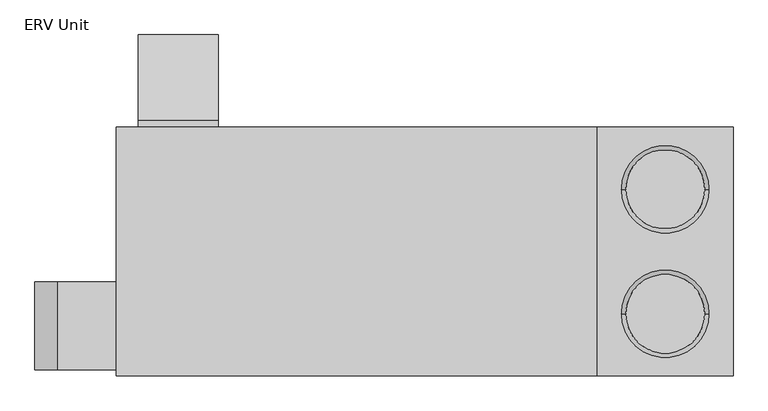
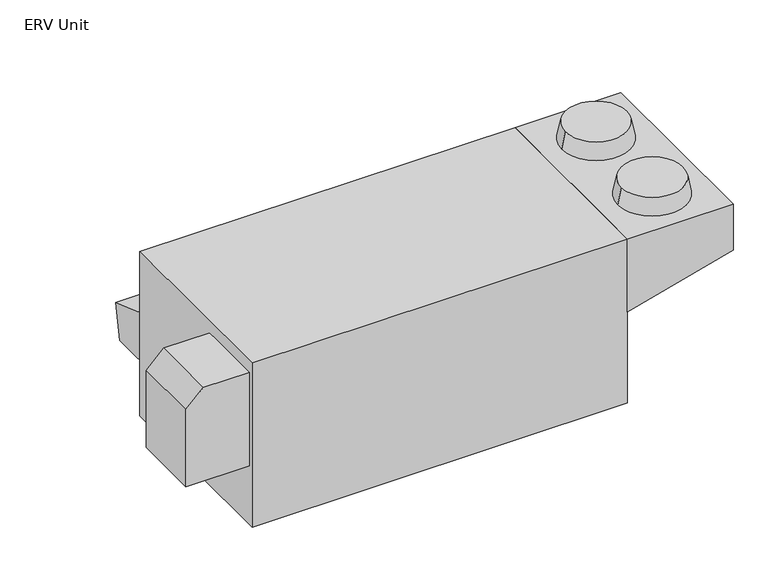
"""IFC4 building model written with IfcOpenShell, lengths in millimetres: proxy geometry, Energy Recovery-ER_H : ERV Unit."""

import ifcopenshell
import ifcopenshell.guid

model = None  # the IFC model being written
_history = None  # IfcOwnerHistory: only IFC2X3 demands one
_inside = {}  # id of a spatial element -> (the spatial element, [elements in it])
_under = {}  # id of a project, library or spatial element -> (it, [spatial elements below it])
_declared = {}  # id of a project -> (the project, [libraries it declares])
_typed = {}  # id of a type object -> (the type object, [elements of that type])
_made_of = {}  # id of a material, layer set ... -> (it, [elements and type objects made of it])


def new_model(schema):
    """Start an empty IFC model of exactly this schema.

    Asked for "IFC4X3", IfcOpenShell would pick the latest addendum, in which some entities
    have other attributes; the version numbers below select the first issue.
    IFC2X3 requires an IfcOwnerHistory on every rooted entity: one is made here for all.
    """
    global model, _history
    if schema == "IFC4X3":
        model = ifcopenshell.file(schema_version=(4, 3, 0, 0))
    else:
        model = ifcopenshell.file(schema=schema)
    _inside.clear()
    _under.clear()
    _declared.clear()
    _typed.clear()
    _made_of.clear()
    _history = None
    if model.schema == "IFC2X3":
        org = make("IfcOrganization", Name="unknown")
        user = make(
            "IfcPersonAndOrganization",
            ThePerson=make("IfcPerson", FamilyName="unknown"),
            TheOrganization=org,
        )
        app = make(
            "IfcApplication",
            ApplicationDeveloper=org,
            Version="unknown",
            ApplicationFullName="unknown",
            ApplicationIdentifier="unknown",
        )
        _history = make(
            "IfcOwnerHistory",
            OwningUser=user,
            OwningApplication=app,
            ChangeAction="ADDED",
            CreationDate=0,
        )
    return model


def make(cls, **values):
    """One entity of the class cls with the attributes given. An attribute that is None is left unset."""
    return model.create_entity(
        cls, **{name: value for name, value in values.items() if value is not None}
    )


def rooted(cls, **values):
    """An entity with a GlobalId (a new one), such as an element, a storey or a relation."""
    return make(cls, GlobalId=ifcopenshell.guid.new(), OwnerHistory=_history, **values)


def si_unit(unit_type, name, prefix=None):
    """IfcSIUnit, for example si_unit("LENGTHUNIT", "METRE", prefix="MILLI")."""
    return make("IfcSIUnit", UnitType=unit_type, Prefix=prefix, Name=name)


def assignment(units):
    """IfcUnitAssignment: the units of a project."""
    return None if units is None else make("IfcUnitAssignment", Units=units)


def point(xyz):
    """IfcCartesianPoint."""
    return None if xyz is None else make("IfcCartesianPoint", Coordinates=xyz)


def direction(xyz):
    """IfcDirection."""
    return None if xyz is None else make("IfcDirection", DirectionRatios=xyz)


def frame(location, z_axis=None, x_axis=None):
    """IfcAxis2Placement3D, a coordinate frame: its origin and axes. An axis left out is left unset."""
    return make(
        "IfcAxis2Placement3D",
        Location=point(location),
        Axis=direction(z_axis),
        RefDirection=direction(x_axis),
    )


def origin():
    """The frame at (0, 0, 0) with its axes left unset."""
    return frame((0.0, 0.0, 0.0))


def place(relative_to, where):
    """IfcLocalPlacement: puts the frame where relative to a parent placement (None: the world)."""
    return make(
        "IfcLocalPlacement", PlacementRelTo=relative_to, RelativePlacement=where
    )


def context(
    kind, dimensions, precision=None, world=None, true_north=None, identifier=None
):
    """IfcGeometricRepresentationContext, for example the 3D "Model" context."""
    return make(
        "IfcGeometricRepresentationContext",
        ContextIdentifier=identifier,
        ContextType=kind,
        CoordinateSpaceDimension=dimensions,
        Precision=precision,
        WorldCoordinateSystem=world,
        TrueNorth=true_north,
    )


def project(units=None, contexts=None):
    """IfcProject with its units and contexts."""
    return rooted(
        "IfcProject",
        Name="project",
        RepresentationContexts=contexts,
        UnitsInContext=assignment(units),
    )


def spatial(cls, under=None, at=None, **own):
    """A site, building, storey or space (cls), placed at a placement, below another one or the project."""
    s = rooted(cls, ObjectPlacement=at, **own)
    if under is not None:
        _under.setdefault(under.id(), (under, []))[1].append(s)
    return s


def polyline(points):
    """IfcPolyline through the points."""
    return make("IfcPolyline", Points=[point(p) for p in points])


def circle_curve(where, radius):
    """IfcCircle in the frame where."""
    return make("IfcCircle", Position=where, Radius=radius)


def outline(outer, holes=None, kind="AREA"):
    """IfcArbitraryClosedProfileDef: a profile drawn as a closed curve; with holes, ...WithVoids."""
    if holes is None:
        return make("IfcArbitraryClosedProfileDef", ProfileType=kind, OuterCurve=outer)
    return make(
        "IfcArbitraryProfileDefWithVoids",
        ProfileType=kind,
        OuterCurve=outer,
        InnerCurves=holes,
    )


def extrude(swept, where, along, depth):
    """IfcExtrudedAreaSolid: the profile swept, set in the frame where, extruded along a direction by depth."""
    return make(
        "IfcExtrudedAreaSolid",
        SweptArea=swept,
        Position=where,
        ExtrudedDirection=direction(along),
        Depth=depth,
    )


def shape(context_of_items, identifier, shape_type, items):
    """IfcShapeRepresentation: the items that make up one representation, for example the "Body"."""
    return make(
        "IfcShapeRepresentation",
        ContextOfItems=context_of_items,
        RepresentationIdentifier=identifier,
        RepresentationType=shape_type,
        Items=items,
    )


def source(mapping_origin, context_of_items, identifier, shape_type, items):
    """IfcRepresentationMap: a shape defined once, which mapped items show again and again."""
    return make(
        "IfcRepresentationMap",
        MappingOrigin=mapping_origin,
        MappedRepresentation=shape(context_of_items, identifier, shape_type, items),
    )


def transform(
    local_origin,
    x_axis=None,
    y_axis=None,
    z_axis=None,
    scale=None,
    scale2=None,
    scale3=None,
    uniform=True,
):
    """IfcCartesianTransformationOperator3D, or its non-uniform kind. x_axis, y_axis, z_axis: its Axis1, 2, 3."""
    if uniform:
        return make(
            "IfcCartesianTransformationOperator3D",
            Axis1=direction(x_axis),
            Axis2=direction(y_axis),
            LocalOrigin=point(local_origin),
            Scale=scale,
            Axis3=direction(z_axis),
        )
    return make(
        "IfcCartesianTransformationOperator3DnonUniform",
        Axis1=direction(x_axis),
        Axis2=direction(y_axis),
        LocalOrigin=point(local_origin),
        Scale=scale,
        Axis3=direction(z_axis),
        Scale2=scale2,
        Scale3=scale3,
    )


def mapped(mapping_source, mapping_target):
    """IfcMappedItem: shows the shape of a source again, moved by a transform."""
    return make(
        "IfcMappedItem", MappingSource=mapping_source, MappingTarget=mapping_target
    )


def made_of(thing, what):
    """Note that an element or type object is made of a material, layer set ...; save() writes the relation."""
    if what is not None:
        _made_of.setdefault(what.id(), (what, []))[1].append(thing)
    return thing


def element(
    cls,
    number,
    at=None,
    inside=None,
    cuts=None,
    type_object=None,
    material=None,
    context=None,
    identifier="Body",
    shape_type=None,
    held_by="IfcProductDefinitionShape",
    body=None,
    shapes=None,
    **own,
):
    """One element of the class cls, such as IfcWall. Its Tag is "e" and its number.

    at: its placement. inside: the storey or other place that contains it. cuts: it is an
    opening in that element (IfcRelVoidsElement). A single representation is given by context,
    identifier, shape_type and body (its items); several are given by shapes. held_by: the class
    of the entity that holds the representations. save() writes the other relations.
    """
    e = rooted(cls, Tag="e%d" % number, ObjectPlacement=at, **own)
    if body is not None:
        shapes = [shape(context, identifier, shape_type, body)]
    if shapes is not None:
        e.Representation = make(held_by, Representations=shapes)
    if inside is not None:
        _inside.setdefault(inside.id(), (inside, []))[1].append(e)
    if cuts is not None:
        rooted(
            "IfcRelVoidsElement", RelatingBuildingElement=cuts, RelatedOpeningElement=e
        )
    if type_object is not None:
        _typed.setdefault(type_object.id(), (type_object, []))[1].append(e)
    return made_of(e, material)


def aggregate(whole, parts):
    """IfcRelAggregates: a whole, such as a stair, and the parts it consists of."""
    return rooted("IfcRelAggregates", RelatingObject=whole, RelatedObjects=parts)


def save(model, path):
    """Write the relations noted so far, then the file.

    IfcRelAggregates (storeys below a building ...), IfcRelContainedInSpatialStructure (elements
    in a storey), IfcRelDefinesByType, IfcRelAssociatesMaterial and IfcRelDeclares: one each for
    every whole, place, type object, material and project.
    """
    for whole, parts in _under.values():
        aggregate(whole, parts)
    for where, things in _inside.values():
        rooted(
            "IfcRelContainedInSpatialStructure",
            RelatedElements=things,
            RelatingStructure=where,
        )
    for kind, things in _typed.values():
        rooted("IfcRelDefinesByType", RelatedObjects=things, RelatingType=kind)
    for what, things in _made_of.values():
        rooted("IfcRelAssociatesMaterial", RelatedObjects=things, RelatingMaterial=what)
    for by, libraries in _declared.values():
        rooted("IfcRelDeclares", RelatingContext=by, RelatedDefinitions=libraries)
    model.write(path)


def plane_surface(at):
    """IfcPlane: the flat surface through the origin of the frame at, square to its z axis."""
    return make("IfcPlane", Position=at)


def revolved_surface(curve, axis_point, axis_direction):
    """IfcSurfaceOfRevolution: the curve turned about the line through axis_point along axis_direction."""
    return make(
        "IfcSurfaceOfRevolution",
        SweptCurve=make("IfcArbitraryOpenProfileDef", ProfileType="CURVE", Curve=curve),
        AxisPosition=make("IfcAxis1Placement", Location=point(axis_point), Axis=direction(axis_direction)),
    )


def advanced_brep(points, edges, surfaces, faces):
    """IfcAdvancedBrep: a solid bounded by faces that lie on surfaces and meet in shared edges.

    An edge is (start, end): straight between two places in points (the first is 0);
    or (start, end, curve); or (start, end, curve, False) where it runs against its curve.
    A face is (place in surfaces, loops), or (place, loops, False) where it looks against
    its surface's normal. A loop lists edges by number (the first is 1), with a minus sign
    where the edge is run from its end to its start. The first loop is the outer one.
    """
    corners = [point(p) for p in points]
    vertices = [make("IfcVertexPoint", VertexGeometry=c) for c in corners]
    made = []
    for start, end, *more in edges:
        made.append(
            make(
                "IfcEdgeCurve",
                EdgeStart=vertices[start],
                EdgeEnd=vertices[end],
                EdgeGeometry=more[0] if more else make("IfcPolyline", Points=[corners[start], corners[end]]),
                SameSense=more[1] if len(more) > 1 else True,
            )
        )
    hull = []
    for where, loops, *sense in faces:
        bounds = []
        for j, loop in enumerate(loops):
            ring = [make("IfcOrientedEdge", EdgeElement=made[abs(k) - 1], Orientation=k > 0) for k in loop]
            bounds.append(
                make(
                    "IfcFaceOuterBound" if j == 0 else "IfcFaceBound",
                    Bound=make("IfcEdgeLoop", EdgeList=ring),
                    Orientation=True,
                )
            )
        hull.append(make("IfcAdvancedFace", Bounds=bounds, FaceSurface=surfaces[where], SameSense=sense[0] if sense else True))
    return make("IfcAdvancedBrep", Outer=make("IfcClosedShell", CfsFaces=hull))


def erv_unit_62530c4e(model_context):
    return source(origin(), model_context, "Body", "SolidModel", [
        extrude(outline(polyline([(740.0249593, 200.025), (740.0249593, 635.0), (778.1249593, 635.0), (1267.0749593, 463.55), (1216.2749593, 200.025), (740.0249593, 200.025)])), frame((-44.3389519, 0.0, 0.0), z_axis=(1.0, 0.0, 0.0), x_axis=(0.0, 1.0, 0.0)), (0.0, 0.0, 1.0), 457.2),
        advanced_brep(
        [(3188.1285481, -326.7750407, 1346.2), (2736.6435481, -326.7750407, 1346.2), (3213.2110481, -326.7750407, 1219.2), (2711.5610481, -326.7750407, 1219.2)],
        [
            (0, 1, circle_curve(frame((2962.3860481, -326.7750407, 1346.2), z_axis=(0.0, 0.0, 1.0), x_axis=(1.0, 0.0, 0.0)), 225.7425)),
            (1, 0, circle_curve(frame((2962.3860481, -326.7750407, 1346.2), z_axis=(0.0, 0.0, 1.0), x_axis=(-1.0, 0.0, 0.0)), 225.7425)),
            (2, 3, circle_curve(frame((2962.3860481, -326.7750407, 1219.2), z_axis=(0.0, 0.0, -1.0), x_axis=(-1.0, 0.0, 0.0)), 250.825)),
            (3, 2, circle_curve(frame((2962.3860481, -326.7750407, 1219.2), z_axis=(0.0, 0.0, -1.0), x_axis=(1.0, 0.0, 0.0)), 250.825)),
            (3, 1),
            (0, 2),
        ],
        [
            plane_surface(frame((2962.3860481, -326.7750407, 1346.2), z_axis=(0.0, 0.0, 1.0), x_axis=(0.0, 1.0, 0.0))),
            plane_surface(frame((2962.3860481, -326.7750407, 1219.2), z_axis=(0.0, 0.0, -1.0), x_axis=(0.0, 1.0, 0.0))),
            revolved_surface(polyline([(3188.1285481, -326.7750407, 1346.2), (3213.2110481, -326.7750407, 1219.2)]), (2962.3860481, -326.7750407, 2489.2), (0.0, 0.0, -1.0)),
            revolved_surface(polyline([(2736.6435481, -326.7750407, 1346.2), (2711.5610481, -326.7750407, 1219.2)]), (2962.3860481, -326.7750407, 2489.2), (0.0, 0.0, -1.0)),
        ],
        [
            (0, [[1, 2]]),
            (1, [[3, 4]]),
            (2, [[-4, 5, -1, 6]]),
            (3, [[-3, -6, -2, -5]]),
        ],
    ),
        advanced_brep(
        [(3188.1285481, 384.4249593, 1346.2), (2736.6435481, 384.4249593, 1346.2), (3213.2110481, 384.4249593, 1219.2), (2711.5610481, 384.4249593, 1219.2)],
        [
            (0, 1, circle_curve(frame((2962.3860481, 384.4249593, 1346.2), z_axis=(0.0, 0.0, 1.0), x_axis=(1.0, 0.0, 0.0)), 225.7425)),
            (1, 0, circle_curve(frame((2962.3860481, 384.4249593, 1346.2), z_axis=(0.0, 0.0, 1.0), x_axis=(-1.0, 0.0, 0.0)), 225.7425)),
            (2, 3, circle_curve(frame((2962.3860481, 384.4249593, 1219.2), z_axis=(0.0, 0.0, -1.0), x_axis=(-1.0, 0.0, 0.0)), 250.825)),
            (3, 2, circle_curve(frame((2962.3860481, 384.4249593, 1219.2), z_axis=(0.0, 0.0, -1.0), x_axis=(1.0, 0.0, 0.0)), 250.825)),
            (3, 1),
            (0, 2),
        ],
        [
            plane_surface(frame((2962.3860481, 384.4249593, 1346.2), z_axis=(0.0, 0.0, 1.0), x_axis=(0.0, 1.0, 0.0))),
            plane_surface(frame((2962.3860481, 384.4249593, 1219.2), z_axis=(0.0, 0.0, -1.0), x_axis=(0.0, 1.0, 0.0))),
            revolved_surface(polyline([(3188.1285481, 384.4249593, 1346.2), (3213.2110481, 384.4249593, 1219.2)]), (2962.3860481, 384.4249593, 2489.2), (0.0, 0.0, -1.0)),
            revolved_surface(polyline([(2736.6435481, 384.4249593, 1346.2), (2711.5610481, 384.4249593, 1219.2)]), (2962.3860481, 384.4249593, 2489.2), (0.0, 0.0, -1.0)),
        ],
        [
            (0, [[1, 2]]),
            (1, [[3, 4]]),
            (2, [[-4, 5, -1, 6]]),
            (3, [[-3, -6, -2, -5]]),
        ],
    ),
        extrude(outline(polyline([(1219.2, 3349.7360481), (1219.2, 2575.0360481), (654.05, 2575.0360481), (863.6, 3349.7360481), (1219.2, 3349.7360481)])), frame((0.0, -682.3750407, 0.0), z_axis=(0.0, 1.0, 0.0), x_axis=(0.0, 0.0, 1.0)), (0.0, 0.0, 1.0), 1422.4),
        extrude(outline(polyline([(403.225, -171.3389519), (1127.125, -171.3389519), (1127.125, -507.8889519), (1000.125, -634.8889519), (403.225, -634.8889519), (403.225, -171.3389519)])), frame((0.0, -647.4500407, 0.0), z_axis=(0.0, 1.0, 0.0), x_axis=(0.0, 0.0, 1.0)), (0.0, 0.0, 1.0), 501.65),
        extrude(outline(polyline([(2060.6860481, 606.6749593), (2060.6860481, 276.4749593), (1425.6860481, 276.4749593), (1425.6860481, 606.6749593), (2060.6860481, 606.6749593)])), frame((0.0, 0.0, -50.8), z_axis=(0.0, 0.0, 1.0), x_axis=(1.0, 0.0, 0.0)), (0.0, 0.0, 1.0), 3.175),
        extrude(outline(polyline([(2194.0360481, -129.9250407), (2194.0360481, -587.1250407), (1838.4360481, -587.1250407), (1838.4360481, -129.9250407), (2194.0360481, -129.9250407)])), frame((0.0, 0.0, -50.8), z_axis=(0.0, 0.0, 1.0), x_axis=(1.0, 0.0, 0.0)), (0.0, 0.0, 1.0), 3.175),
        extrude(outline(polyline([(2575.0360481, 740.0249593), (2575.0360481, -682.3750407), (-171.3389519, -682.3750407), (-171.3389519, 740.0249593), (2575.0360481, 740.0249593)])), frame((0.0, 0.0, -50.8), z_axis=(0.0, 0.0, 1.0), x_axis=(1.0, 0.0, 0.0)), (0.0, 0.0, 1.0), 1270.0),
    ])


if __name__ == "__main__":
    model = new_model("IFC4")
    model_context = context("Model", 3, world=origin())
    ifc_project = project(units=[si_unit("LENGTHUNIT", "METRE", prefix="MILLI")], contexts=[model_context])
    site = spatial("IfcSite", under=ifc_project)
    building = spatial("IfcBuilding", under=site)
    placement = place(None, origin())
    erv_unit_shape = erv_unit_62530c4e(model_context)
    element("IfcBuildingElementProxy", 1, Name="Energy Recovery-ER_H : ERV Unit", ObjectType="Energy Recovery-ER_H : ERV Unit", at=placement, inside=building, context=model_context, shape_type="MappedRepresentation", body=[
        mapped(erv_unit_shape, transform((0.0, 0.0, 0.0), x_axis=(1.0, 0.0, 0.0), y_axis=(0.0, 1.0, 0.0), z_axis=(0.0, 0.0, 1.0))),
    ])
    save(model, "model.ifc")

# Revit data of these elements
# Type "Energy Recovery-ER_H : ERV Unit"
#   Version Family = "rfa 1.0 Beta"
#   Version Data = "NA"
#   URL = "http://www.greenheck.com/products/detail/51"
#   Tag = ""
#   Supply Filter = ""
#   OAI Weatherhood End Description = "Louvered Outdoor Air Intake"
#   OAI Duct Top Description = "Alternative connector is used"
#   OAI Duct End Description = "Alternative connector is used"
#   OAD Duct Top Description = "Alternative connector is used"
#   OAD Duct Side Description = "Alternative connector is used"
#   OAD Duct End Description = "Alternative connector is used"
#   OAD Duct Bottom Description = "Supply Air Discharge"
#   Model = "ERCH-20M-15"
#   Manufacturing Location = "United States"
#   Manufacturer = "Greenheck"
#   Invalid Connector = "Alternative connector is used"
#   Exhaust Filter = ""
#   Energy Wheel Model = "0"
#   EAI Duct Top Description = "Alternative connector is used"
#   EAI Duct Bottom Description = "Exhaust Air Intake"
#   EAI Duct Back Description = "Alternative connector is used"
#   EAD Weatherhood Side Description = "Side Exhaust Air Weatherhood"
#   EAD Weatherhood End Description = "Alternative connector is used"
#   EAD Duct Top Description = "Alternative connector is used"
#   EAD Duct Side Description = "Alternative connector is used"
#   EAD Duct End Description = "Alternative connector is used"
#   Description = "Energy Recovery with Cooling & Heating"
#   Copyright © = "© Greenheck Fan Corp 2009"
#   Configured Mark Name = "ERV Unit"
#   Voltage = 460 V
#   Unit Weight = 0.0000625 kip
#   Supply Static Pressure = 0.00 in-wg
#   Supply Air Flow Rate = 1400 CFM
#   PDX Length = 2' - 6 1/2"
#   PDX Front Height = 1' - 2"
#   PDX Cooling Radius Top = 0' - 8.8875"
#   PDX Cooling Radius = 0' - 9 7/8"
#   PDX Back Height = 1' - 10 1/4"
#   OAI Half Depth = 0' - 9 1/8"
#   OAI Duct Width = 1' - 7 3/4"
#   OAI Duct Vert = 2' - 8 1/8"
#   OAI Duct Horiz = 0' - 11 1/4"
#   OAI Duct Height = 2' - 4 1/2"
#   OAI Depth = 1' - 6 1/4"
#   OAD Duct Width = 1' - 6"
#   OAD Duct Vert = 1' - 10"
#   OAD Duct Horiz = 1' - 0 3/4"
#   OAD Duct Height = 1' - 2"
#   Length PDX = 2' - 6"
#   IG Heater Width = 2' - 7"
#   IG Heater Offset = 0' - 1"
#   IG Heater Height = 0' - 0"
#   IG Heater Height NZ = 0' - 1"
#   IG Heater Depth = 0' - 10"
#   Half Under Sizing = 0' - 1"
#   Exhaust Static Pressure = 0.00 in-wg
#   Exhaust Air Flow Rate = 1400 CFM
#   Energy Wheel Depth = 0' - 1 1/2"
#   Electrical Load = 0 VA
#   Electrical Current = 60 Hz
#   EAI Duct Width = 1' - 1"
#   EAI Duct Vert = 2' - 8 3/4"
#   EAI Duct Horiz = 0' - 11 3/4"
#   EAI Duct Height = 2' - 1"
#   EAD Duct Width = 1' - 6"
#   EAD Duct Vert = 1' - 8 1/4"
#   EAD Duct Horiz = 1' - 2"
#   EAD Duct Height = 1' - 5 1/8"
#   EAD Depth = 1' - 8 3/4"
#   CurbWidth = 4' - 6"
#   CurbLength = 8' - 10 1/8"
#   Curb Under Sizing = 0' - 2"
#   Curb Height = 0' - 1"
#   Base Width = 4' - 8"
#   Base Length = 9' - 0 1/8"
#   Base Height = 4' - 2"
#   Apparent Load = 0 VA
#   VFD = no
#   Roof Curb = no
#   Phase = 3
#   Packaged DX = yes
#   OAI Weatherhood End = yes
#   OAI Duct Top = no
#   OAI Duct End = no
#   OAD Duct Top = no
#   OAD Duct Side = no
#   OAD Duct Bottom = yes
#   OAD Duct End = no
#   Number of Poles = 3
#   Indirect Gas Heater = yes
#   IG Heater Top = no
#   IG Heater Bottom = no
#   Has Special Design = no
#   EAI Duct Top = no
#   EAI Duct Bottom = yes
#   EAI Duct Back = no
#   EAD Weatherhood Side = yes
#   EAD Weatherhood End = no
#   EAD Duct Top = no
#   EAD Duct End = no
#   EAD Duct Side = no
#   Load Classification = HVAC
#   Type Comments = ""
#   Default Elevation = 0
#   Assembly Code = ""
